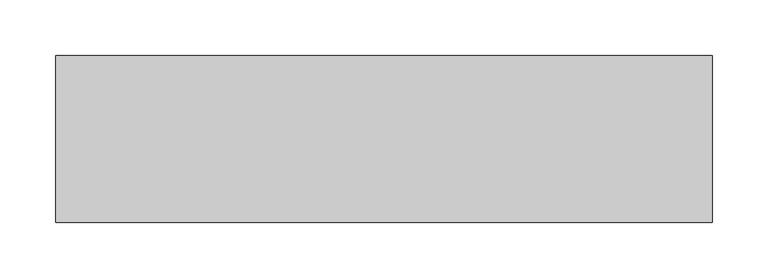
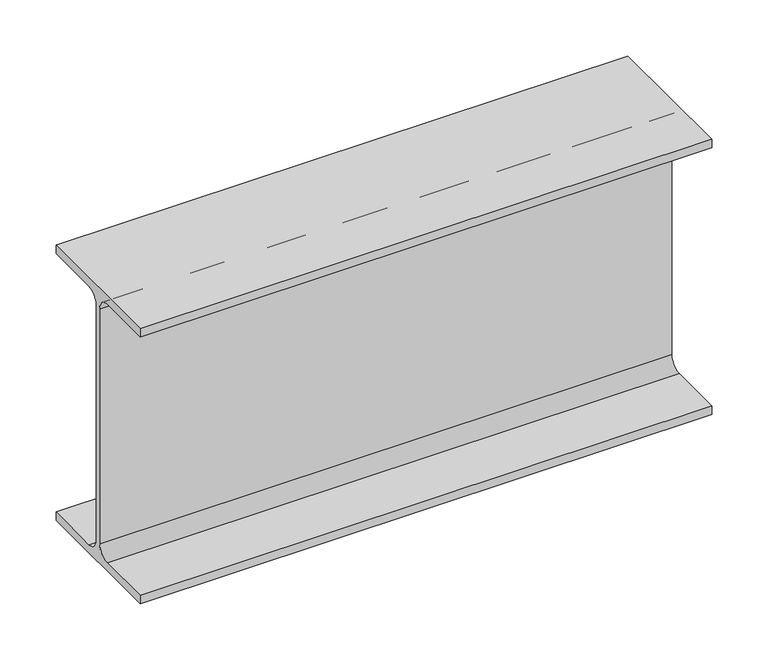
"""IFC4 building model written with IfcOpenShell, lengths in millimetres: beam geometry, 0912_Steel Framing_H-KSD3502 : H_SB_ASB_H-300x150x6.5x9."""

from ifc_helpers import new_model, si_unit, point, frame, frame_2d, origin, place, context, project, spatial, polyline, circle_curve, trimmed, segment, composite_curve, outline, extrude, source, transform, mapped, element, save


def beam_b6fb0ee1(model_context):
    return source(origin(), model_context, "Body", "SweptSolid", [
        extrude(outline(composite_curve([segment(polyline([(75.0, -141.0), (75.0, -150.0), (-75.0, -150.0), (-75.0, -141.0), (-16.25, -141.0)]), True, "CONTINUOUS"), segment(trimmed(circle_curve(frame_2d((-16.25, -128.0)), 13.0), [point((-16.25, -141.0))], [point((-3.25, -128.0))], True, "CARTESIAN"), True, "CONTINUOUS"), segment(polyline([(-3.25, -128.0), (-3.25, 128.0)]), True, "CONTINUOUS"), segment(trimmed(circle_curve(frame_2d((-16.25, 128.0)), 13.0), [point((-3.25, 128.0))], [point((-16.25, 141.0))], True, "CARTESIAN"), True, "CONTINUOUS"), segment(polyline([(-16.25, 141.0), (-75.0, 141.0), (-75.0, 150.0), (75.0, 150.0), (75.0, 141.0), (16.25, 141.0)]), True, "CONTINUOUS"), segment(trimmed(circle_curve(frame_2d((16.25, 128.0)), 13.0), [point((16.25, 141.0))], [point((3.25, 128.0))], True, "CARTESIAN"), True, "CONTINUOUS"), segment(polyline([(3.25, 128.0), (3.25, -128.0)]), True, "CONTINUOUS"), segment(trimmed(circle_curve(frame_2d((16.25, -128.0)), 13.0), [point((3.25, -128.0))], [point((16.25, -141.0))], True, "CARTESIAN"), True, "CONTINUOUS"), segment(polyline([(16.25, -141.0), (75.0, -141.0)]), True, "CONTINUOUS")], self_intersect=False)), frame((-282.3, 0.0, 0.0), z_axis=(1.0, 0.0, 0.0), x_axis=(0.0, 1.0, 0.0)), (0.0, 0.0, 1.0), 589.6),
    ])


if __name__ == "__main__":
    model = new_model("IFC4")
    model_context = context("Model", 3, world=origin())
    ifc_project = project(units=[si_unit("LENGTHUNIT", "METRE", prefix="MILLI")], contexts=[model_context])
    site = spatial("IfcSite", under=ifc_project)
    building = spatial("IfcBuilding", under=site)
    placement = place(None, origin())
    beam_shape = beam_b6fb0ee1(model_context)
    element("IfcBeam", 1, ObjectType="0912_Steel Framing_H-KSD3502 : H_SB_ASB_H-300x150x6.5x9", at=placement, inside=building, context=model_context, shape_type="MappedRepresentation", body=[
        mapped(beam_shape, transform((0.0, 0.0, 0.0), x_axis=(1.0, 0.0, 0.0), y_axis=(0.0, 1.0, 0.0), z_axis=(0.0, 0.0, 1.0))),
    ])
    save(model, "model.ifc")

# Revit data of these elements
# Type "0912_Steel Framing_H-KSD3502 : H_SB_ASB_H-300x150x6.5x9"
#   H_WM Code_1 = "S01AA002-00001 | Main Steel Structure Fabrication Work | Shelter/Building | Medium Steel - Standard (90KG/M>Weight≥30KG/M) | Material: (   )"
#   H_WM Code_2 = "S03AA028-00001 | Main Steel Structure Erection Work | Shelter/Building | Medium Steel (90KG/M>Weight≥30KG/M) | Material: (   )"
#   H_WM Code_3 = "S01AA010-00001 | Main Steel Structure Fabrication Work | Shelter/Building | Steel Painting/Coating | for Non-Fireproofed Steel Surface, Surface Preparation, Primer, Second & Final Coat | Material: (   )"
#   H_Q'ty Cal Type Tag = "SB-Q2"
#   Width = 15.0 cm
#   Web Thickness = 0.65 cm
#   Web Fillet = 1.3 cm
#   Warping Constant = 107000.0 cm⁶
#   W = 0
#   Torsional Moment of Inertia = 9.9539 cm⁴
#   Section Area = 46.78 cm²
#   Plastic Modulus weak axis = 105.0 cm³
#   Plastic Modulus strong axis = 542.0 cm³
#   Perimeter = 1.17 m²/m
#   Nominal Weight = 36.70 kgf/m
#   Moment of Inertia weak axis = 508.00 cm⁴
#   Moment of Inertia strong axis = 7210.00 cm⁴
#   Height = 30.0 cm
#   Flange Thickness = 0.9 cm
#   Elastic Modulus weak axis = 67.7 cm³
#   Elastic Modulus strong axis = 481.0 cm³
#   Centroid Vertical = 15.0 cm
#   Centroid Horizontal = 7.5 cm
#   Ix = 72100000
#   Length [instance default] = 1.5240 m
#   Zx = 542000
#   b = 0.1500 m
#   h = 0.3000 m
#   r = 0.0130 m
#   s = 0.0065 m
#   t = 0.0090 m
#   A = 0.004678 m²
#   Structural Material [instance default] = Steel, 45-345
#   Assembly Code = ""
# Element 1 (IfcBeam, "0912_Steel Framing_H-KSD3502 : H_SB_ASB_H-300x150x6.5x9")
#   Structural Material = none
# Materials
#   "Steel, 45-345": class "Metal", colour RGB 189 187 185, transparency 0, Description = "Steel 345 MPa", Cost = 0
